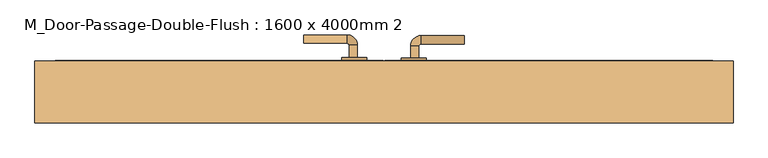
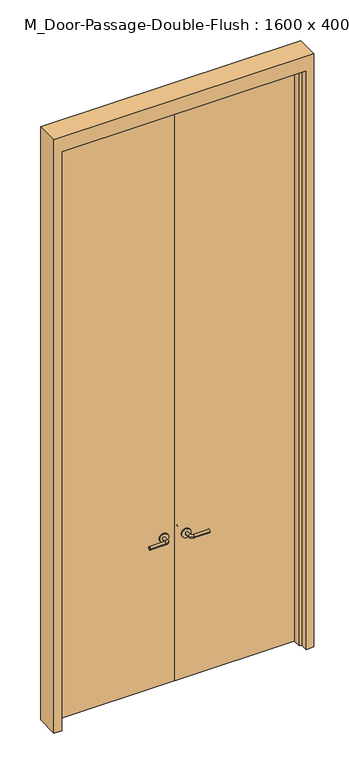
"""IFC4 building model written with IfcOpenShell, lengths in millimetres: door geometry, M_Door-Passage-Double-Flush : 1600 x 4000mm 2."""

from ifc_helpers import new_model, si_unit, point, frame, frame_2d, origin, origin_with_axes, place, context, project, spatial, polyline, circle_curve, ellipse_curve, trimmed, segment, composite_curve, outline, extrude, faceted_brep, source, transform, mapped, element, save
from ifc_brep_helpers import plane_surface, cylinder_surface, revolved_surface, advanced_brep


def m_door_passage_double_flush_1600_x_4000mm_2_a9a1b764(model_context):
    return source(origin(), model_context, "Body", "SolidModel", [
        advanced_brep(
        [(-65.009375, 28.35, 1016.0), (-85.009375, 28.35, 1016.0), (-65.009375, -1.65, 1016.0), (-85.009375, -1.65, 1016.0), (-90.009375, -6.65, 1016.0), (-90.009375, -26.65, 1016.0), (-195.009375, -26.65, 1016.0), (-195.009375, -6.65, 1016.0)],
        [
            (0, 1, circle_curve(frame((-75.009375, 28.35, 1016.0), z_axis=(0.0, 1.0, 0.0), x_axis=(-1.0, 0.0, 0.0)), 10.0)),
            (1, 0, circle_curve(frame((-75.009375, 28.35, 1016.0), z_axis=(0.0, 1.0, 0.0), x_axis=(-1.0, 0.0, 0.0)), 10.0)),
            (0, 2),
            (2, 3, circle_curve(frame((-75.009375, -1.65, 1016.0), z_axis=(0.0, 1.0, 0.0), x_axis=(-1.0, 0.0, 0.0)), 10.0)),
            (3, 1),
            (3, 2, circle_curve(frame((-75.009375, -1.65, 1016.0), z_axis=(0.0, 1.0, 0.0), x_axis=(-1.0, 0.0, 0.0)), 10.0)),
            (4, 3, circle_curve(frame((-90.009375, -1.65, 1016.0), z_axis=(0.0, 0.0, 1.0), x_axis=(1.0, 0.0, 0.0)), 5.0)),
            (2, 5, circle_curve(frame((-90.009375, -1.65, 1016.0), z_axis=(0.0, 0.0, -1.0), x_axis=(1.0, 0.0, 0.0)), 25.0)),
            (5, 4, circle_curve(frame((-90.009375, -16.65, 1016.0), z_axis=(1.0, 0.0, 0.0), x_axis=(0.0, 1.0, 0.0)), 10.0)),
            (4, 5, circle_curve(frame((-90.009375, -16.65, 1016.0), z_axis=(1.0, 0.0, 0.0), x_axis=(0.0, 1.0, 0.0)), 10.0)),
            (6, 7, circle_curve(frame((-195.009375, -16.65, 1016.0), z_axis=(-1.0, 0.0, 0.0), x_axis=(0.0, 1.0, 0.0)), 10.0)),
            (7, 6, circle_curve(frame((-195.009375, -16.65, 1016.0), z_axis=(-1.0, 0.0, 0.0), x_axis=(0.0, 1.0, 0.0)), 10.0)),
            (5, 6),
            (7, 4),
        ],
        [
            plane_surface(frame((-75.009375, 28.35, 1016.0), z_axis=(0.0, 1.0, 0.0), x_axis=(0.0, 0.0, 1.0))),
            cylinder_surface(frame((-75.009375, 28.35, 1016.0), z_axis=(0.0, 1.0, 0.0), x_axis=(-1.0, 0.0, 0.0)), 10.0),
            revolved_surface(trimmed(ellipse_curve(frame((-75.009375, -1.65, 1016.0), z_axis=(0.0, 1.0, 0.0), x_axis=(-1.0, 0.0, 0.0)), 10.0, 10.0), [point((-65.009375, -1.65, 1016.0))], [point((-85.009375, -1.65, 1016.0))], True, "CARTESIAN"), (-90.009375, -1.65, 1016.0), (0.0, 0.0, -1.0)),
            revolved_surface(trimmed(ellipse_curve(frame((-75.009375, -1.65, 1016.0), z_axis=(0.0, 1.0, 0.0), x_axis=(-1.0, 0.0, 0.0)), 10.0, 10.0), [point((-85.009375, -1.65, 1016.0))], [point((-65.009375, -1.65, 1016.0))], True, "CARTESIAN"), (-90.009375, -1.65, 1016.0), (0.0, 0.0, -1.0)),
            plane_surface(frame((-195.009375, -16.65, 1016.0), z_axis=(-1.0, 0.0, 0.0), x_axis=(0.0, 0.0, 1.0))),
            cylinder_surface(frame((-90.009375, -16.65, 1016.0), z_axis=(1.0, 0.0, 0.0), x_axis=(0.0, 1.0, 0.0)), 10.0),
        ],
        [
            (0, [[1, 2]]),
            (1, [[-1, 3, 4, 5]]),
            (1, [[-2, -5, 6, -3]]),
            (2, [[7, -4, 8, 9]]),
            (3, [[-8, -6, -7, 10]]),
            (4, [[11, 12]]),
            (5, [[-9, 13, -12, 14]]),
            (5, [[-10, -14, -11, -13]]),
        ],
    ),
        extrude(outline(composite_curve([segment(trimmed(circle_curve(frame_2d((1016.0, -72.509375)), 30.0), [point((1016.0, -42.509375))], [point((1016.0, -102.509375))], False, "CARTESIAN"), True, "CONTINUOUS"), segment(trimmed(circle_curve(frame_2d((1016.0, -72.509375)), 30.0), [point((1016.0, -102.509375))], [point((1016.0, -42.509375))], False, "CARTESIAN"), True, "CONTINUOUS")], self_intersect=False)), frame((0.0, 28.35, 0.0), z_axis=(0.0, 1.0, 0.0), x_axis=(0.0, 0.0, 1.0)), (0.0, 0.0, 1.0), 8.0),
        advanced_brep(
        [(-65.009375, 90.95, 1000.0), (-85.009375, 90.95, 1000.0), (-85.009375, 120.95, 1000.0), (-65.009375, 120.95, 1000.0), (-90.009375, 125.95, 1000.0), (-90.009375, 145.95, 1000.0), (-195.009375, 145.95, 1000.0), (-195.009375, 125.95, 1000.0)],
        [
            (0, 1, circle_curve(frame((-75.009375, 90.95, 1000.0), z_axis=(0.0, -1.0, 0.0), x_axis=(-1.0, 0.0, 0.0)), 10.0)),
            (1, 0, circle_curve(frame((-75.009375, 90.95, 1000.0), z_axis=(0.0, -1.0, 0.0), x_axis=(-1.0, 0.0, 0.0)), 10.0)),
            (1, 2),
            (2, 3, circle_curve(frame((-75.009375, 120.95, 1000.0), z_axis=(0.0, -1.0, 0.0), x_axis=(-1.0, 0.0, 0.0)), 10.0)),
            (3, 0),
            (3, 2, circle_curve(frame((-75.009375, 120.95, 1000.0), z_axis=(0.0, -1.0, 0.0), x_axis=(-1.0, 0.0, 0.0)), 10.0)),
            (4, 5, circle_curve(frame((-90.009375, 135.95, 1000.0), z_axis=(1.0, 0.0, 0.0), x_axis=(0.0, -1.0, 0.0)), 10.0)),
            (5, 3, circle_curve(frame((-90.009375, 120.95, 1000.0), z_axis=(0.0, 0.0, -1.0), x_axis=(1.0, 0.0, 0.0)), 25.0)),
            (2, 4, circle_curve(frame((-90.009375, 120.95, 1000.0), z_axis=(0.0, 0.0, 1.0), x_axis=(1.0, 0.0, 0.0)), 5.0)),
            (5, 4, circle_curve(frame((-90.009375, 135.95, 1000.0), z_axis=(1.0, 0.0, 0.0), x_axis=(0.0, -1.0, 0.0)), 10.0)),
            (6, 7, circle_curve(frame((-195.009375, 135.95, 1000.0), z_axis=(-1.0, 0.0, 0.0), x_axis=(0.0, -1.0, 0.0)), 10.0)),
            (7, 6, circle_curve(frame((-195.009375, 135.95, 1000.0), z_axis=(-1.0, 0.0, 0.0), x_axis=(0.0, -1.0, 0.0)), 10.0)),
            (4, 7),
            (6, 5),
        ],
        [
            plane_surface(frame((-75.009375, 90.95, 1000.0), z_axis=(0.0, -1.0, 0.0), x_axis=(0.0, 0.0, 1.0))),
            cylinder_surface(frame((-75.009375, 90.95, 1000.0), z_axis=(0.0, -1.0, 0.0), x_axis=(-1.0, 0.0, 0.0)), 10.0),
            revolved_surface(trimmed(ellipse_curve(frame((-75.009375, 120.95, 1000.0), z_axis=(0.0, 1.0, 0.0), x_axis=(-1.0, 0.0, 0.0)), 10.0, 10.0), [point((-65.009375, 120.95, 1000.0))], [point((-85.009375, 120.95, 1000.0))], True, "CARTESIAN"), (-90.009375, 120.95, 1000.0), (0.0, 0.0, -1.0)),
            revolved_surface(trimmed(ellipse_curve(frame((-75.009375, 120.95, 1000.0), z_axis=(0.0, 1.0, 0.0), x_axis=(-1.0, 0.0, 0.0)), 10.0, 10.0), [point((-85.009375, 120.95, 1000.0))], [point((-65.009375, 120.95, 1000.0))], True, "CARTESIAN"), (-90.009375, 120.95, 1000.0), (0.0, 0.0, -1.0)),
            plane_surface(frame((-195.009375, 135.95, 1000.0), z_axis=(-1.0, 0.0, 0.0), x_axis=(0.0, 0.0, 1.0))),
            cylinder_surface(frame((-90.009375, 135.95, 1000.0), z_axis=(1.0, 0.0, 0.0), x_axis=(0.0, -1.0, 0.0)), 10.0),
        ],
        [
            (0, [[1, 2]]),
            (1, [[3, 4, 5, -2]]),
            (1, [[-5, 6, -3, -1]]),
            (2, [[7, 8, -4, 9]]),
            (3, [[10, -9, -6, -8]]),
            (4, [[11, 12]]),
            (5, [[13, -11, 14, -7]]),
            (5, [[-14, -12, -13, -10]]),
        ],
    ),
        extrude(outline(composite_curve([segment(trimmed(circle_curve(frame_2d((1000.0, -72.509375)), 30.0), [point((1000.0, -42.509375))], [point((1000.0, -102.509375))], False, "CARTESIAN"), True, "CONTINUOUS"), segment(trimmed(circle_curve(frame_2d((1000.0, -72.509375)), 30.0), [point((1000.0, -102.509375))], [point((1000.0, -42.509375))], False, "CARTESIAN"), True, "CONTINUOUS")], self_intersect=False)), frame((0.0, 82.95, 0.0), z_axis=(0.0, 1.0, 0.0), x_axis=(0.0, 0.0, 1.0)), (0.0, 0.0, 1.0), 8.0),
        advanced_brep(
        [(65.009375, 28.35, 1000.0), (85.009375, 28.35, 1000.0), (85.009375, -1.65, 1000.0), (65.009375, -1.65, 1000.0), (90.009375, -6.65, 1000.0), (90.009375, -26.65, 1000.0), (195.009375, -26.65, 1000.0), (195.009375, -6.65, 1000.0)],
        [
            (0, 1, circle_curve(frame((75.009375, 28.35, 1000.0), z_axis=(0.0, 1.0, 0.0), x_axis=(1.0, 0.0, 0.0)), 10.0)),
            (1, 0, circle_curve(frame((75.009375, 28.35, 1000.0), z_axis=(0.0, 1.0, 0.0), x_axis=(1.0, 0.0, 0.0)), 10.0)),
            (1, 2),
            (2, 3, circle_curve(frame((75.009375, -1.65, 1000.0), z_axis=(0.0, 1.0, 0.0), x_axis=(1.0, 0.0, 0.0)), 10.0)),
            (3, 0),
            (3, 2, circle_curve(frame((75.009375, -1.65, 1000.0), z_axis=(0.0, 1.0, 0.0), x_axis=(1.0, 0.0, 0.0)), 10.0)),
            (4, 5, circle_curve(frame((90.009375, -16.65, 1000.0), z_axis=(-1.0, 0.0, 0.0), x_axis=(0.0, 1.0, 0.0)), 10.0)),
            (5, 3, circle_curve(frame((90.009375, -1.65, 1000.0), z_axis=(0.0, 0.0, -1.0), x_axis=(-1.0, 0.0, 0.0)), 25.0)),
            (2, 4, circle_curve(frame((90.009375, -1.65, 1000.0), z_axis=(0.0, 0.0, 1.0), x_axis=(-1.0, 0.0, 0.0)), 5.0)),
            (5, 4, circle_curve(frame((90.009375, -16.65, 1000.0), z_axis=(-1.0, 0.0, 0.0), x_axis=(0.0, 1.0, 0.0)), 10.0)),
            (6, 7, circle_curve(frame((195.009375, -16.65, 1000.0), z_axis=(1.0, 0.0, 0.0), x_axis=(0.0, 1.0, 0.0)), 10.0)),
            (7, 6, circle_curve(frame((195.009375, -16.65, 1000.0), z_axis=(1.0, 0.0, 0.0), x_axis=(0.0, 1.0, 0.0)), 10.0)),
            (4, 7),
            (6, 5),
        ],
        [
            plane_surface(frame((75.009375, 28.35, 1000.0), z_axis=(0.0, 1.0, 0.0), x_axis=(0.0, 0.0, 1.0))),
            cylinder_surface(frame((75.009375, 28.35, 1000.0), z_axis=(0.0, 1.0, 0.0), x_axis=(1.0, 0.0, 0.0)), 10.0),
            revolved_surface(trimmed(ellipse_curve(frame((75.009375, -1.65, 1000.0), z_axis=(0.0, -1.0, 0.0), x_axis=(1.0, 0.0, 0.0)), 10.0, 10.0), [point((65.009375, -1.65, 1000.0))], [point((85.009375, -1.65, 1000.0))], True, "CARTESIAN"), (90.009375, -1.65, 1000.0), (0.0, 0.0, -1.0)),
            revolved_surface(trimmed(ellipse_curve(frame((75.009375, -1.65, 1000.0), z_axis=(0.0, -1.0, 0.0), x_axis=(1.0, 0.0, 0.0)), 10.0, 10.0), [point((85.009375, -1.65, 1000.0))], [point((65.009375, -1.65, 1000.0))], True, "CARTESIAN"), (90.009375, -1.65, 1000.0), (0.0, 0.0, -1.0)),
            plane_surface(frame((195.009375, -16.65, 1000.0), z_axis=(1.0, 0.0, 0.0), x_axis=(0.0, 0.0, 1.0))),
            cylinder_surface(frame((90.009375, -16.65, 1000.0), z_axis=(-1.0, 0.0, 0.0), x_axis=(0.0, 1.0, 0.0)), 10.0),
        ],
        [
            (0, [[1, 2]]),
            (1, [[3, 4, 5, -2]]),
            (1, [[-5, 6, -3, -1]]),
            (2, [[7, 8, -4, 9]]),
            (3, [[10, -9, -6, -8]]),
            (4, [[11, 12]]),
            (5, [[13, -11, 14, -7]]),
            (5, [[-14, -12, -13, -10]]),
        ],
    ),
        extrude(outline(composite_curve([segment(trimmed(circle_curve(frame_2d((1000.0, 72.509375)), 30.0), [point((1000.0, 42.509375))], [point((1000.0, 102.509375))], False, "CARTESIAN"), True, "CONTINUOUS"), segment(trimmed(circle_curve(frame_2d((1000.0, 72.509375)), 30.0), [point((1000.0, 102.509375))], [point((1000.0, 42.509375))], False, "CARTESIAN"), True, "CONTINUOUS")], self_intersect=False)), frame((0.0, 28.35, 0.0), z_axis=(0.0, 1.0, 0.0), x_axis=(0.0, 0.0, 1.0)), (0.0, 0.0, 1.0), 8.0),
        advanced_brep(
        [(65.009375, 89.35, 1000.0), (85.009375, 89.35, 1000.0), (65.009375, 119.35, 1000.0), (85.009375, 119.35, 1000.0), (90.009375, 124.35, 1000.0), (90.009375, 144.35, 1000.0), (195.009375, 144.35, 1000.0), (195.009375, 124.35, 1000.0)],
        [
            (0, 1, circle_curve(frame((75.009375, 89.35, 1000.0), z_axis=(0.0, -1.0, 0.0), x_axis=(1.0, 0.0, 0.0)), 10.0)),
            (1, 0, circle_curve(frame((75.009375, 89.35, 1000.0), z_axis=(0.0, -1.0, 0.0), x_axis=(1.0, 0.0, 0.0)), 10.0)),
            (0, 2),
            (2, 3, circle_curve(frame((75.009375, 119.35, 1000.0), z_axis=(0.0, -1.0, 0.0), x_axis=(1.0, 0.0, 0.0)), 10.0)),
            (3, 1),
            (3, 2, circle_curve(frame((75.009375, 119.35, 1000.0), z_axis=(0.0, -1.0, 0.0), x_axis=(1.0, 0.0, 0.0)), 10.0)),
            (4, 3, circle_curve(frame((90.009375, 119.35, 1000.0), z_axis=(0.0, 0.0, 1.0), x_axis=(-1.0, 0.0, 0.0)), 5.0)),
            (2, 5, circle_curve(frame((90.009375, 119.35, 1000.0), z_axis=(0.0, 0.0, -1.0), x_axis=(-1.0, 0.0, 0.0)), 25.0)),
            (5, 4, circle_curve(frame((90.009375, 134.35, 1000.0), z_axis=(-1.0, 0.0, 0.0), x_axis=(0.0, -1.0, 0.0)), 10.0)),
            (4, 5, circle_curve(frame((90.009375, 134.35, 1000.0), z_axis=(-1.0, 0.0, 0.0), x_axis=(0.0, -1.0, 0.0)), 10.0)),
            (6, 7, circle_curve(frame((195.009375, 134.35, 1000.0), z_axis=(1.0, 0.0, 0.0), x_axis=(0.0, -1.0, 0.0)), 10.0)),
            (7, 6, circle_curve(frame((195.009375, 134.35, 1000.0), z_axis=(1.0, 0.0, 0.0), x_axis=(0.0, -1.0, 0.0)), 10.0)),
            (5, 6),
            (7, 4),
        ],
        [
            plane_surface(frame((75.009375, 89.35, 1000.0), z_axis=(0.0, -1.0, 0.0), x_axis=(0.0, 0.0, 1.0))),
            cylinder_surface(frame((75.009375, 89.35, 1000.0), z_axis=(0.0, -1.0, 0.0), x_axis=(1.0, 0.0, 0.0)), 10.0),
            revolved_surface(trimmed(ellipse_curve(frame((75.009375, 119.35, 1000.0), z_axis=(0.0, -1.0, 0.0), x_axis=(1.0, 0.0, 0.0)), 10.0, 10.0), [point((65.009375, 119.35, 1000.0))], [point((85.009375, 119.35, 1000.0))], True, "CARTESIAN"), (90.009375, 119.35, 1000.0), (0.0, 0.0, -1.0)),
            revolved_surface(trimmed(ellipse_curve(frame((75.009375, 119.35, 1000.0), z_axis=(0.0, -1.0, 0.0), x_axis=(1.0, 0.0, 0.0)), 10.0, 10.0), [point((85.009375, 119.35, 1000.0))], [point((65.009375, 119.35, 1000.0))], True, "CARTESIAN"), (90.009375, 119.35, 1000.0), (0.0, 0.0, -1.0)),
            plane_surface(frame((195.009375, 134.35, 1000.0), z_axis=(1.0, 0.0, 0.0), x_axis=(0.0, 0.0, 1.0))),
            cylinder_surface(frame((90.009375, 134.35, 1000.0), z_axis=(-1.0, 0.0, 0.0), x_axis=(0.0, -1.0, 0.0)), 10.0),
        ],
        [
            (0, [[1, 2]]),
            (1, [[-1, 3, 4, 5]]),
            (1, [[-2, -5, 6, -3]]),
            (2, [[7, -4, 8, 9]]),
            (3, [[-8, -6, -7, 10]]),
            (4, [[11, 12]]),
            (5, [[-9, 13, -12, 14]]),
            (5, [[-10, -14, -11, -13]]),
        ],
    ),
        extrude(outline(composite_curve([segment(trimmed(circle_curve(frame_2d((1000.0, 72.509375)), 30.0), [point((1000.0, 42.509375))], [point((1000.0, 102.509375))], False, "CARTESIAN"), True, "CONTINUOUS"), segment(trimmed(circle_curve(frame_2d((1000.0, 72.509375)), 30.0), [point((1000.0, 102.509375))], [point((1000.0, 42.509375))], False, "CARTESIAN"), True, "CONTINUOUS")], self_intersect=False)), frame((0.0, 81.35, 0.0), z_axis=(0.0, 1.0, 0.0), x_axis=(0.0, 0.0, 1.0)), (0.0, 0.0, 1.0), 8.0),
        extrude(outline(polyline([(800.0, 36.35), (1.5875, 36.35), (1.5875, 82.95), (800.0, 82.95), (800.0, 36.35)])), origin_with_axes(), (0.0, 0.0, 1.0), 4000.0),
        extrude(outline(polyline([(-1.5875, 36.35), (-800.0, 36.35), (-800.0, 82.95), (-1.5875, 82.95), (-1.5875, 36.35)])), origin_with_axes(), (0.0, 0.0, 1.0), 4000.0),
        faceted_brep([(800.0, 31.5875, 0.0), (800.0, 81.35, 0.0), (850.0, 81.35, 0.0), (850.0, -68.65, 0.0), (800.0, -68.65, 0.0), (800.0, -19.4375, 0.0), (784.125, -19.4375, 0.0), (784.125, 31.5875, 0.0), (800.0, 31.5875, 4000.0), (800.0, 81.35, 4000.0), (-800.0, 81.35, 4000.0), (-800.0, 81.35, 0.0), (-850.0, 81.35, 0.0), (-850.0, 81.35, 4100.0), (850.0, 81.35, 4100.0), (850.0, -68.65, 4100.0), (-850.0, -68.65, 4100.0), (-850.0, -68.65, 0.0), (-800.0, -68.65, 0.0), (-800.0, -68.65, 4000.0), (800.0, -68.65, 4000.0), (800.0, -19.4375, 4000.0), (-800.0, -19.4375, 4000.0), (-800.0, -19.4375, 0.0), (-784.125, -19.4375, 0.0), (-784.125, -19.4375, 3984.125), (784.125, -19.4375, 3984.125), (784.125, 31.5875, 3984.125), (-784.125, 31.5875, 3984.125), (-784.125, 31.5875, 0.0), (-800.0, 31.5875, 0.0), (-800.0, 31.5875, 4000.0)], [[[0, 1, 2, 3, 4, 5, 6, 7]], [[1, 0, 8, 9]], [[2, 1, 9, 10, 11, 12, 13, 14]], [[3, 2, 14, 15]], [[4, 3, 15, 16, 17, 18, 19, 20]], [[5, 4, 20, 21]], [[6, 5, 21, 22, 23, 24, 25, 26]], [[7, 6, 26, 27]], [[0, 7, 27, 28, 29, 30, 31, 8]], [[9, 8, 31, 10]], [[20, 19, 22, 21]], [[26, 25, 28, 27]], [[12, 11, 30, 29, 24, 23, 18, 17]], [[11, 10, 31, 30]], [[13, 12, 17, 16]], [[19, 18, 23, 22]], [[25, 24, 29, 28]], [[15, 14, 13, 16]]]),
    ])


if __name__ == "__main__":
    model = new_model("IFC4")
    model_context = context("Model", 3, world=origin())
    ifc_project = project(units=[si_unit("LENGTHUNIT", "METRE", prefix="MILLI")], contexts=[model_context])
    site = spatial("IfcSite", under=ifc_project)
    building = spatial("IfcBuilding", under=site)
    placement = place(None, origin())
    m_door_passage_double_flush_1600_x_4000mm_2_shape = m_door_passage_double_flush_1600_x_4000mm_2_a9a1b764(model_context)
    element("IfcDoor", 1, ObjectType="M_Door-Passage-Double-Flush : 1600 x 4000mm 2", at=placement, inside=building, context=model_context, shape_type="MappedRepresentation", body=[
        mapped(m_door_passage_double_flush_1600_x_4000mm_2_shape, transform((0.0, 0.0, 0.0), x_axis=(1.0, 0.0, 0.0), y_axis=(0.0, 1.0, 0.0), z_axis=(0.0, 0.0, 1.0))),
    ])
    save(model, "model.ifc")

# Revit data of these elements
# Type "M_Door-Passage-Double-Flush : 1600 x 4000mm 2"
#   Type Mark = "46"
#   Analytic Construction = "Metal"
#   Thickness = 45 mm
#   Thermal Resistance (R) = 0.270118 (m²·K)/W
#   Swing Angle [instance default] = 90.00°
#   Strike Height = 1000 mm
#   SinglePanelWidth = 800 mm
#   Rough Width [instance default] = 1700 mm
#   Rough Height [instance default] = 4100 mm
#   MFOpeningHeight [instance default] = 100 mm
#   MFOpeningWidth [instance default] = 100 mm
#   Inset Calculate [instance default] = 105 mm
#   Masonry Inset [instance default] = 25 mm
#   Height = 4000 mm
#   Width = 1600 mm
#   Heat Transfer Coefficient (U) = 3.70223 W/(m²·K)
#   Masonry Frame Depth = 150 mm
#   Masonry Frame [instance default] = yes
#   Function = 1
#   Dry Wall Frame [instance default] = no
#   Panel Material = Glass, Clear Glazing
#   Frame Material = Metal - Painted - Grey
#   Door Handle Material = Aluminum
#   Visual Light Transmittance = 0
#   Solar Heat Gain Coefficient = 0
#   Wall Closure = (empty or 0)
# Element 1 (IfcDoor, "M_Door-Passage-Double-Flush : 1600 x 4000mm 2")
#   Materials on its faces: "Aluminum", "Metal - Painted - Grey", "Glass, Clear Glazing"
# Materials
#   "Glass, Clear Glazing": class "Glass", colour RGB 223 223 223, transparency 1, Description = "Clear glazing", Cost = 0
#   "Metal - Painted - Grey": class "Paint", colour RGB 104 104 104, transparency 0
#   "Aluminum": class "Metal", colour RGB 244 245 246, transparency 0, Description = "Aluminum 6061", Cost = 0
